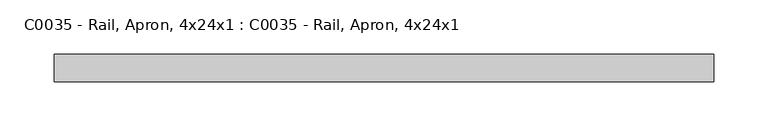
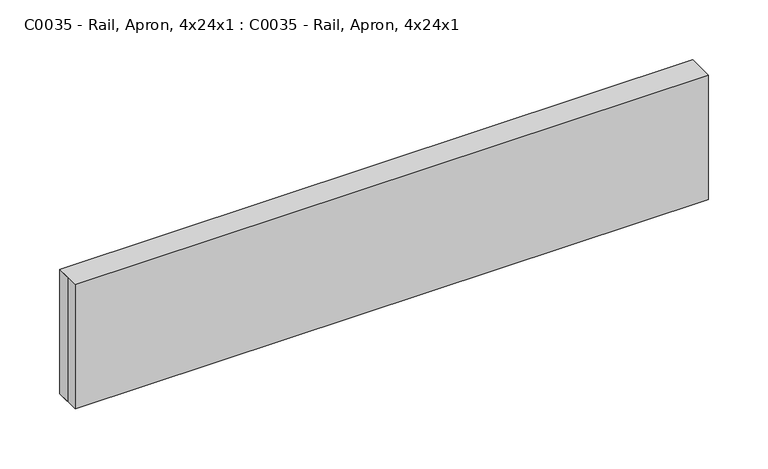
"""IFC4 building model written with IfcOpenShell, lengths in millimetres: proxy geometry, C0035 - Rail, Apron, 4x24x1 : C0035 - Rail, Apron, 4x24x1."""

from ifc_helpers import new_model, si_unit, origin, origin_with_axes, place, context, project, spatial, polyline, outline, extrude, source, transform, mapped, element, save


def c0035_rail_apron_4x24x1_c0035_rail_apron_4x24x1_13c9656f(model_context):
    return source(origin(), model_context, "Body", "SweptSolid", [
        extrude(outline(polyline([(-304.8, 12.7), (304.8, 12.7), (304.8, -12.7), (-304.8, -12.7), (-304.8, 0.0), (-304.8, 12.7)])), origin_with_axes(), (0.0, 0.0, 1.0), 127.0),
        extrude(outline(polyline([(304.8, -12.7), (-304.8, -12.7), (-304.8, 12.7), (304.8, 12.7), (304.8, -12.7)])), origin_with_axes(), (0.0, 0.0, 1.0), 127.0),
    ])


if __name__ == "__main__":
    model = new_model("IFC4")
    model_context = context("Model", 3, world=origin())
    ifc_project = project(units=[si_unit("LENGTHUNIT", "METRE", prefix="MILLI")], contexts=[model_context])
    site = spatial("IfcSite", under=ifc_project)
    building = spatial("IfcBuilding", under=site)
    placement = place(None, origin())
    c0035_rail_apron_4x24x1_c0035_rail_apron_4x24x1_shape = c0035_rail_apron_4x24x1_c0035_rail_apron_4x24x1_13c9656f(model_context)
    element("IfcBuildingElementProxy", 1, Name="C0035 - Rail, Apron, 4x24x1 : C0035 - Rail, Apron, 4x24x1", ObjectType="C0035 - Rail, Apron, 4x24x1 : C0035 - Rail, Apron, 4x24x1", at=placement, inside=building, context=model_context, shape_type="MappedRepresentation", body=[
        mapped(c0035_rail_apron_4x24x1_c0035_rail_apron_4x24x1_shape, transform((0.0, 0.0, 0.0), x_axis=(1.0, 0.0, 0.0), y_axis=(0.0, 1.0, 0.0), z_axis=(0.0, 0.0, 1.0))),
    ])
    save(model, "model.ifc")

# Revit data of these elements
# Project information
#   Room Abbreviation = "DNTS1"
#   Room Description = "Dental Treatment Room, Oral Surgery (DNTS1)"
#   Sheets - Total = "5"
#   Project Issue Date = "Issue Date"
#   Project Status = "Project Status"
#   Client Name = "Owner"
#   Project Address = "Enter address here"
#   Project Name = "Project Name"
#   Project Number = "Project Number"
#   Publication Date = "30-Jan-15"
# Type "C0035 - Rail, Apron, 4x24x1 : C0035 - Rail, Apron, 4x24x1"
#   Watts2 = "0"
#   Watts1 = "0"
#   Unit_Issue = "EA"
#   UTIL_6_Misc = "-"
#   UTIL_5_NonMedGas = "-"
#   UTIL_4_MiscGas = "-"
#   UTIL_3_MedGas = "-"
#   UTIL_2_Elec = "-"
#   UTIL_1_WaterDrain = "-"
#   Nomenclature = "Rail, Apron, 4x24x1"
#   NSN = "6530"
#   Location [instance default] = ""
#   JSN = "C0035"
#   Fund_Source_VA = "-"
#   Fund_Source_Navy = "-"
#   Fund_Source_Army = "-"
#   Fund_Source_AF = "-"
#   ELEC_Volts2 = "0"
#   ELEC_Volts1 = "0"
#   ELEC_Phase2 = "0"
#   ELEC_Phase1 = "0"
#   ELEC_HertzSwitch = "0"
#   ELEC_HertzDependent = "0"
#   ELEC_Hertz = "0"
#   ELEC_Amps2 = "0"
#   ELEC_Amps1 = "0"
#   DetailDescription = "Apron rail. Also referred to as an apron front, apron panel, or knee space rail. Used to close in front knee space area and/or provide work surface support between two base cabinets or a base cabinet and wall. Apron rails should be ordered in pairs to provide both front and rear work surface support."
#   CAT_VA = "A"
#   CAT_Navy = "A"
#   CAT_IHS = "-"
#   CAT_Army = "A"
#   CAT_AF = "A"
#   BTUperhour = "0"
#   Weight_IP = 7
#   DIM_Width_IP = 2' - 0"
#   DIM_Height_IP = 0' - 5"
#   DIM_Depth_IP = 0' - 1"
#   Top Panel Material = none
#   Toe Panel Material = none
#   Side Panel Material = none
#   Shelf Panel Material = none
#   Drawer Front Material = none
#   Door Panel Material = none
#   Back Panel Material = none
#   Assembly Code = ""
# Element 1 (IfcBuildingElementProxy, "C0035 - Rail, Apron, 4x24x1 : C0035 - Rail, Apron, 4x24x1")
#   Materials on its faces: "EquipSpace"
# Materials
#   "EquipSpace": class "Unassigned", colour RGB 221 217 195, transparency 0.5
